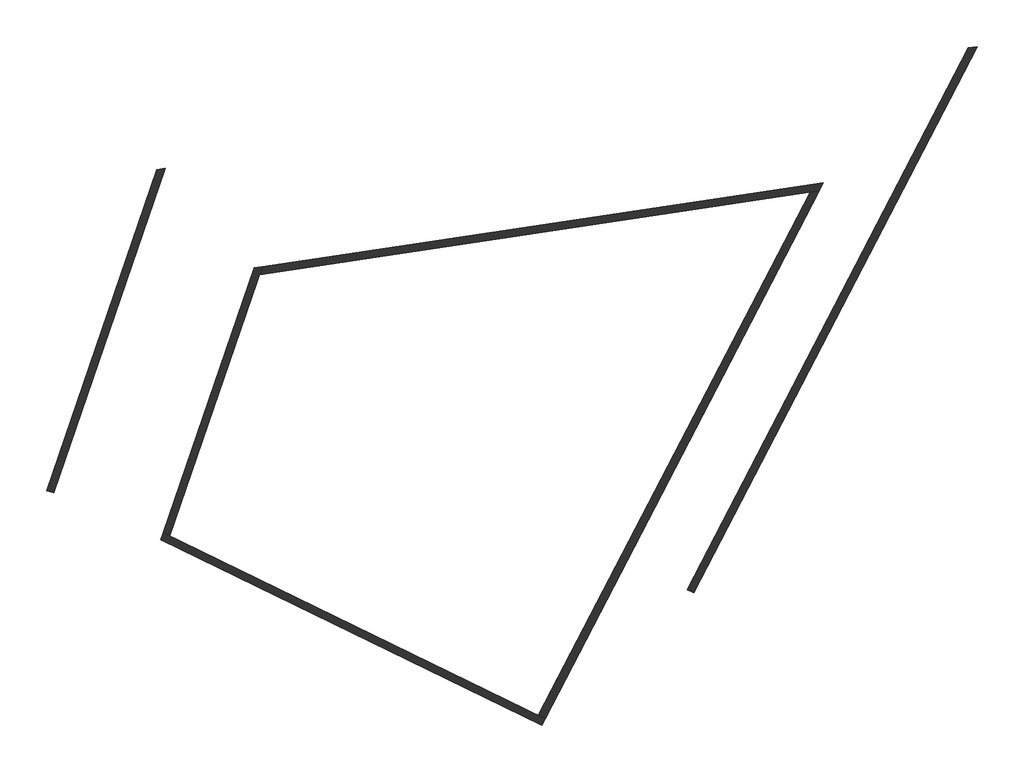
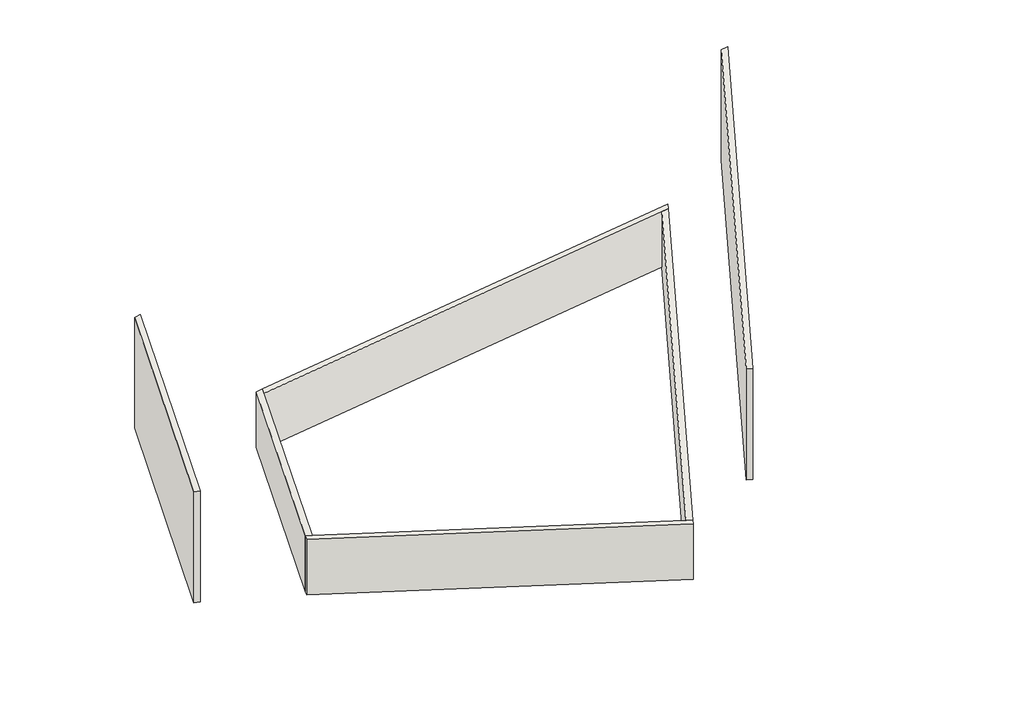
# One storey: 6 walls.
"""IFC4 building model written with IfcOpenShell, lengths in millimetres."""

from ifc_helpers import new_model, si_unit, frame, origin, place, context, project, spatial, polyline, outline, extrude, faceted_brep, element, save

model = new_model("IFC4")

# Units and contexts
model_context = context("Model", 3, world=origin())
ifc_project = project(units=[si_unit("LENGTHUNIT", "METRE", prefix="MILLI")], contexts=[model_context])

# Site, building, storey
site = spatial("IfcSite", under=ifc_project)
building = spatial("IfcBuilding", under=site)
storey = spatial("IfcBuildingStorey", under=building, Name="Çekme Alanı", Elevation=6000.0)

# Walls
placement = place(None, origin())
element("IfcWall", 1, ObjectType="Generic - 300mm Masonry", at=placement, inside=storey, context=model_context, shape_type="Brep", body=[
    faceted_brep([(99267.9390909, 49133.0090218, 6000.0), (114693.1643825, 41618.7174909, 6000.0), (114693.1643825, 41618.7174909, 9000.0), (99267.9390909, 49133.0090218, 9000.0), (99366.2617944, 49418.8148897, 6000.0), (99366.2617944, 49418.8148897, 9000.0), (99637.9813419, 49286.4485964, 9000.0), (114561.6077302, 42016.5074927, 9000.0), (114831.395489, 41885.0822569, 9000.0), (114831.395489, 41885.0822569, 6000.0), (114561.6077302, 42016.5074927, 6000.0), (99637.9813419, 49286.4485964, 6000.0)], [[[0, 1, 2, 3]], [[4, 5, 6, 7, 8, 9, 10, 11]], [[1, 0, 4, 11, 10, 9]], [[3, 2, 8, 7, 6, 5]], [[0, 3, 5, 4]], [[2, 1, 9, 8]]]),
])
element("IfcWall", 2, ObjectType="Generic - 300mm Masonry", at=placement, inside=storey, context=model_context, shape_type="Brep", body=[
    faceted_brep([(99637.9813419, 49286.4485964, 6000.0), (103277.4815183, 59865.8007732, 6000.0), (103387.5201942, 60185.6628008, 6000.0), (103387.5201942, 60185.6628008, 9000.0), (103277.4815183, 59865.8007732, 9000.0), (99637.9813419, 49286.4485964, 9000.0), (99366.2617944, 49418.8148897, 6000.0), (99366.2617944, 49418.8148897, 9000.0), (103053.0019998, 60135.4850716, 9000.0), (103053.0019998, 60135.4850716, 6000.0)], [[[0, 1, 2, 3, 4, 5]], [[6, 7, 8, 9]], [[2, 1, 0, 6, 9]], [[5, 4, 3, 8, 7]], [[0, 5, 7, 6]], [[3, 2, 9, 8]]]),
])
element("IfcWall", 3, ObjectType="Generic - 300mm Masonry", at=placement, inside=storey, context=model_context, shape_type="Brep", body=[
    faceted_brep([(103277.4815183, 59865.8007732, 6000.0), (125559.0390197, 63208.0343984, 6000.0), (125925.5617259, 63263.0128043, 6000.0), (125925.5617259, 63263.0128043, 9000.0), (125559.0390197, 63208.0343984, 9000.0), (103277.4815183, 59865.8007732, 9000.0), (103387.5201942, 60185.6628008, 6000.0), (103387.5201942, 60185.6628008, 9000.0), (126096.2788604, 63591.9766007, 9000.0), (126096.2788604, 63591.9766007, 6000.0)], [[[0, 1, 2, 3, 4, 5]], [[6, 7, 8, 9]], [[2, 1, 0, 6, 9]], [[5, 4, 3, 8, 7]], [[0, 5, 7, 6]], [[3, 2, 9, 8]]]),
])
element("IfcWall", 4, ObjectType="Generic - 300mm Masonry", at=placement, inside=storey, context=model_context, shape_type="SweptSolid", body=[
    extrude(outline(polyline([(114561.6077302, 42016.5074927), (125559.0390197, 63208.0343984), (125925.5617259, 63263.0128043), (114831.395489, 41885.0822569), (114561.6077302, 42016.5074927)])), frame((0.0, 0.0, 6000.0), z_axis=(0.0, 0.0, 1.0), x_axis=(1.0, 0.0, 0.0)), (0.0, 0.0, 1.0), 3000.0),
])
element("IfcWall", 5, ObjectType="Generic - 300mm Masonry", at=placement, inside=storey, context=model_context, shape_type="Brep", body=[
    faceted_brep([(120853.4406232, 46975.1391138, 6000.0), (132333.7510951, 69097.1512317, 6000.0), (132333.7510951, 69097.1512317, 9000.0), (132333.7510951, 69097.1512317, 12000.0), (120853.4406232, 46975.1391138, 12000.0), (120587.1616848, 47113.3256796, 6000.0), (120587.1616848, 47113.3256796, 12000.0), (131967.2283888, 69042.1728257, 12000.0), (131967.2283888, 69042.1728257, 6000.0)], [[[0, 1, 2, 3, 4]], [[5, 6, 7, 8]], [[1, 0, 5, 8]], [[4, 3, 7, 6]], [[0, 4, 6, 5]], [[3, 2, 1, 8, 7]]]),
])
element("IfcWall", 6, ObjectType="Generic - 300mm Masonry", at=placement, inside=storey, context=model_context, shape_type="Brep", body=[
    faceted_brep([(94928.2113625, 51022.200248, 6000.0), (99449.4149698, 64164.5008129, 6000.0), (99449.4149698, 64164.5008129, 12000.0), (94928.2113625, 51022.200248, 12000.0), (94928.2113625, 51022.200248, 9000.0), (94644.5288673, 51119.7924705, 6000.0), (94644.5288673, 51119.7924705, 9000.0), (94644.5288673, 51119.7924705, 12000.0), (99114.8967753, 64114.3230837, 12000.0), (99114.8967753, 64114.3230837, 9000.0), (99114.8967753, 64114.3230837, 6000.0)], [[[0, 1, 2, 3, 4]], [[5, 6, 7, 8, 9, 10]], [[1, 0, 5, 10]], [[3, 2, 8, 7]], [[0, 4, 3, 7, 6, 5]], [[2, 1, 10, 9, 8]]]),
])

save(model, "model.ifc")

# Revit data of these elements
# Project information
#   Organization Name = "Organization Name"
#   Organization Description = "Organization Description"
#   Building Name = "Building Name"
#   Project Issue Date = "Issue Date"
#   Project Status = "Project Status"
#   Client Name = "Client Name"
#   Project Address = "Enter address here\nAddress Line 2"
#   Project Name = "Project Name"
#   Project Number = "Project Number"
# Type "Generic - 300mm Masonry"
#   Description = "Generic Wall (Material By Category), 300mm thick, Masonry pattern"
#   Assembly Code = "B2010"
#   Type Mark = "G10"
#   Layers, outside or top first: 30 cm "Gravel" (function 1)
# Elements 1, 2, 3, 4 (IfcWall, "Generic - 300mm Masonry")
#   Top Offset = 0 cm
#   Base Offset = 0 cm
#   wall height = 300 cm
#   Phase Created = New Construction
#   Base Constraint = Çekme Alanı
#   Top Constraint = Bodrum Kat
#   Materials on its faces: "Gravel"
# Elements 5, 6 (IfcWall, "Generic - 300mm Masonry")
#   Top Offset = 0 cm
#   Base Offset = 0 cm
#   wall height = 600 cm
#   Phase Created = New Construction
#   Base Constraint = Çekme Alanı
#   Top Constraint = Zemin Kat
#   Materials on its faces: "Gravel"
# Materials
#   "Gravel": class "Generic", colour RGB 120 120 120, transparency 0, Description = "Crushed stone or gravel", Cost = 0
